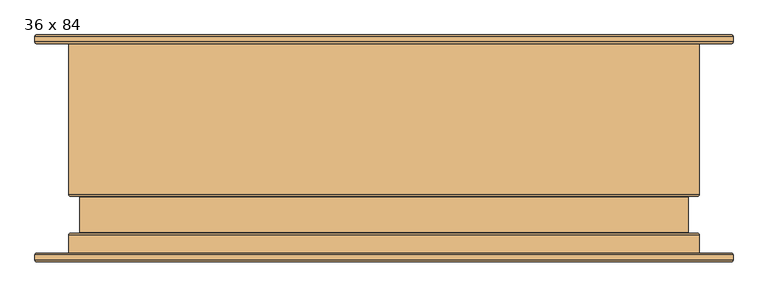
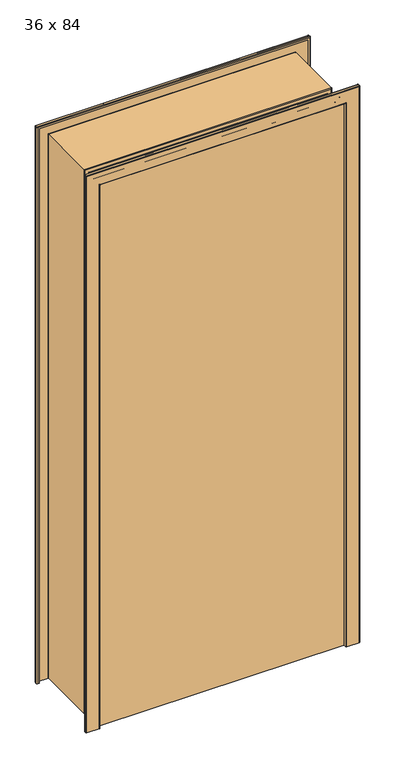
"""IFC4 building model written with IfcOpenShell, lengths in millimetres: door geometry, Door-Dunbarton_Doors-Hollow_Metal_Core : 36 x 84."""

from ifc_helpers import new_model, si_unit, frame, origin, origin_with_axes, place, context, project, spatial, polyline, circle_curve, ellipse_curve, outline, extrude, source, transform, mapped, element, save
from ifc_brep_helpers import plane_surface, cylinder_surface, revolved_surface, advanced_brep


def door_36_x_84_2b1949fa(model_context):
    return source(origin(), model_context, "Body", "SolidModel", [
        advanced_brep(
        [(-505.42825, 152.4635, 0.0), (-508.0, 155.03525, 0.0), (-508.0, 162.56, 0.0), (-505.42825, 165.13175, 0.0), (-459.77175, 165.13175, 0.0), (-457.2, 162.56, 0.0), (-457.2, -67.21475, 0.0), (-456.184, -68.23075, 0.0), (-443.89675, -68.23075, 0.0), (-441.325, -70.8025, 0.0), (-441.325, -122.5931, 0.0), (-443.89675, -125.16485, 0.0), (-456.184, -125.16485, 0.0), (-457.2, -126.18085, 0.0), (-457.2, -162.4965, 0.0), (-459.77175, -165.06825, 0.0), (-505.42825, -165.06825, 0.0), (-508.0, -162.4965, 0.0), (-508.0, -154.97175, 0.0), (-505.42825, -152.4, 0.0), (-500.0625, -152.4, 0.0), (-500.0625, -153.95575, 0.0), (-505.42825, -153.95575, 0.0), (-506.44425, -154.97175, 0.0), (-506.44425, -162.4965, 0.0), (-505.42825, -163.5125, 0.0), (-459.77175, -163.5125, 0.0), (-458.75575, -162.4965, 0.0), (-458.75575, -126.18085, 0.0), (-456.184, -123.6091, 0.0), (-443.89675, -123.6091, 0.0), (-442.88075, -122.5931, 0.0), (-442.88075, -70.8025, 0.0), (-443.89675, -69.7865, 0.0), (-456.184, -69.7865, 0.0), (-458.75575, -67.21475, 0.0), (-458.75575, 162.56, 0.0), (-459.77175, 163.576, 0.0), (-505.42825, 163.576, 0.0), (-506.44425, 162.56, 0.0), (-506.44425, 155.03525, 0.0), (-505.42825, 154.01925, 0.0), (-500.0625, 154.01925, 0.0), (-500.0625, 152.4635, 0.0), (-505.42825, 152.4635, 2181.82825), (-508.0, 155.03525, 2184.4), (-508.0, 162.56, 2184.4), (-505.42825, 165.13175, 2181.82825), (505.42825, 165.13175, 2181.82825), (505.42825, 165.13175, 0.0), (459.77175, 165.13175, 0.0), (459.77175, 165.13175, 2136.17175), (-459.77175, 165.13175, 2136.17175), (-457.2, 162.56, 2133.6), (-457.2, -67.21475, 2133.6), (-456.184, -68.23075, 2132.584), (456.184, -68.23075, 2132.584), (456.184, -68.23075, 0.0), (443.89675, -68.23075, 0.0), (443.89675, -68.23075, 2120.29675), (-443.89675, -68.23075, 2120.29675), (-441.325, -70.8025, 2117.725), (-441.325, -122.5931, 2117.725), (-443.89675, -125.16485, 2120.29675), (443.89675, -125.16485, 2120.29675), (443.89675, -125.16485, 0.0), (456.184, -125.16485, 0.0), (456.184, -125.16485, 2132.584), (-456.184, -125.16485, 2132.584), (-457.2, -126.18085, 2133.6), (-457.2, -162.4965, 2133.6), (-459.77175, -165.06825, 2136.17175), (459.77175, -165.06825, 2136.17175), (459.77175, -165.06825, 0.0), (505.42825, -165.06825, 0.0), (505.42825, -165.06825, 2181.82825), (-505.42825, -165.06825, 2181.82825), (-508.0, -162.4965, 2184.4), (-508.0, -154.97175, 2184.4), (-505.42825, -152.4, 2181.82825), (505.42825, -152.4, 2181.82825), (505.42825, -152.4, 0.0), (500.0625, -152.4, 0.0), (500.0625, -152.4, 2176.4625), (-500.0625, -152.4, 2176.4625), (-500.0625, -153.95575, 2176.4625), (500.0625, -153.95575, 2176.4625), (500.0625, -153.95575, 0.0), (505.42825, -153.95575, 0.0), (505.42825, -153.95575, 2181.82825), (-505.42825, -153.95575, 2181.82825), (-506.44425, -154.97175, 2182.84425), (-506.44425, -162.4965, 2182.84425), (-505.42825, -163.5125, 2181.82825), (505.42825, -163.5125, 2181.82825), (505.42825, -163.5125, 0.0), (459.77175, -163.5125, 0.0), (459.77175, -163.5125, 2136.17175), (-459.77175, -163.5125, 2136.17175), (-458.75575, -162.4965, 2135.15575), (-458.75575, -126.18085, 2135.15575), (-456.184, -123.6091, 2132.584), (456.184, -123.6091, 2132.584), (456.184, -123.6091, 0.0), (443.89675, -123.6091, 0.0), (443.89675, -123.6091, 2120.29675), (-443.89675, -123.6091, 2120.29675), (-442.88075, -122.5931, 2119.28075), (-442.88075, -70.8025, 2119.28075), (-443.89675, -69.7865, 2120.29675), (443.89675, -69.7865, 2120.29675), (443.89675, -69.7865, 0.0), (456.184, -69.7865, 0.0), (456.184, -69.7865, 2132.584), (-456.184, -69.7865, 2132.584), (-458.75575, -67.21475, 2135.15575), (-458.75575, 162.56, 2135.15575), (-459.77175, 163.576, 2136.17175), (459.77175, 163.576, 2136.17175), (459.77175, 163.576, 0.0), (505.42825, 163.576, 0.0), (505.42825, 163.576, 2181.82825), (-505.42825, 163.576, 2181.82825), (-506.44425, 162.56, 2182.84425), (-506.44425, 155.03525, 2182.84425), (-505.42825, 154.01925, 2181.82825), (505.42825, 154.01925, 2181.82825), (505.42825, 154.01925, 0.0), (500.0625, 154.01925, 0.0), (500.0625, 154.01925, 2176.4625), (-500.0625, 154.01925, 2176.4625), (-500.0625, 152.4635, 2176.4625), (500.0625, 152.4635, 2176.4625), (500.0625, 152.4635, 0.0), (505.42825, 152.4635, 0.0), (505.42825, 152.4635, 2181.82825), (508.0, 155.03525, 2184.4), (508.0, 162.56, 2184.4), (457.2, 162.56, 2133.6), (457.2, -67.21475, 2133.6), (441.325, -70.8025, 2117.725), (441.325, -122.5931, 2117.725), (457.2, -126.18085, 2133.6), (457.2, -162.4965, 2133.6), (508.0, -162.4965, 2184.4), (508.0, -154.97175, 2184.4), (506.44425, -154.97175, 2182.84425), (506.44425, -162.4965, 2182.84425), (458.75575, -162.4965, 2135.15575), (458.75575, -126.18085, 2135.15575), (442.88075, -122.5931, 2119.28075), (442.88075, -70.8025, 2119.28075), (458.75575, -67.21475, 2135.15575), (458.75575, 162.56, 2135.15575), (506.44425, 162.56, 2182.84425), (506.44425, 155.03525, 2182.84425), (506.44425, 155.03525, 0.0), (506.44425, 162.56, 0.0), (458.75575, 162.56, 0.0), (458.75575, -67.21475, 0.0), (442.88075, -70.8025, 0.0), (442.88075, -122.5931, 0.0), (458.75575, -126.18085, 0.0), (458.75575, -162.4965, 0.0), (506.44425, -162.4965, 0.0), (506.44425, -154.97175, 0.0), (508.0, -154.97175, 0.0), (508.0, -162.4965, 0.0), (457.2, -162.4965, 0.0), (457.2, -126.18085, 0.0), (441.325, -122.5931, 0.0), (441.325, -70.8025, 0.0), (457.2, -67.21475, 0.0), (457.2, 162.56, 0.0), (508.0, 162.56, 0.0), (508.0, 155.03525, 0.0)],
        [
            (0, 1, circle_curve(frame((-505.42825, 155.03525, 0.0), z_axis=(0.0, 0.0, -1.0), x_axis=(0.0, -1.0, 0.0)), 2.57175)),
            (1, 2),
            (2, 3, circle_curve(frame((-505.42825, 162.56, 0.0), z_axis=(0.0, 0.0, -1.0), x_axis=(0.0, -1.0, 0.0)), 2.57175)),
            (3, 4),
            (4, 5, circle_curve(frame((-459.77175, 162.56, 0.0), z_axis=(0.0, 0.0, -1.0), x_axis=(0.0, -1.0, 0.0)), 2.57175)),
            (5, 6),
            (6, 7, circle_curve(frame((-456.184, -67.21475, 0.0), z_axis=(0.0, 0.0, 1.0), x_axis=(0.0, -1.0, 0.0)), 1.016)),
            (7, 8),
            (8, 9, circle_curve(frame((-443.89675, -70.8025, 0.0), z_axis=(0.0, 0.0, -1.0), x_axis=(0.0, -1.0, 0.0)), 2.57175)),
            (9, 10),
            (10, 11, circle_curve(frame((-443.89675, -122.5931, 0.0), z_axis=(0.0, 0.0, -1.0), x_axis=(0.0, -1.0, 0.0)), 2.57175)),
            (11, 12),
            (12, 13, circle_curve(frame((-456.184, -126.18085, 0.0), z_axis=(0.0, 0.0, 1.0), x_axis=(0.0, -1.0, 0.0)), 1.016)),
            (13, 14),
            (14, 15, circle_curve(frame((-459.77175, -162.4965, 0.0), z_axis=(0.0, 0.0, -1.0), x_axis=(0.0, -1.0, 0.0)), 2.57175)),
            (15, 16),
            (16, 17, circle_curve(frame((-505.42825, -162.4965, 0.0), z_axis=(0.0, 0.0, -1.0), x_axis=(0.0, -1.0, 0.0)), 2.57175)),
            (17, 18),
            (18, 19, circle_curve(frame((-505.42825, -154.97175, 0.0), z_axis=(0.0, 0.0, -1.0), x_axis=(0.0, -1.0, 0.0)), 2.57175)),
            (19, 20),
            (20, 21),
            (21, 22),
            (22, 23, circle_curve(frame((-505.42825, -154.97175, 0.0), z_axis=(0.0, 0.0, 1.0), x_axis=(0.0, -1.0, 0.0)), 1.016)),
            (23, 24),
            (24, 25, circle_curve(frame((-505.42825, -162.4965, 0.0), z_axis=(0.0, 0.0, 1.0), x_axis=(0.0, -1.0, 0.0)), 1.016)),
            (25, 26),
            (26, 27, circle_curve(frame((-459.77175, -162.4965, 0.0), z_axis=(0.0, 0.0, 1.0), x_axis=(0.0, -1.0, 0.0)), 1.016)),
            (27, 28),
            (28, 29, circle_curve(frame((-456.184, -126.18085, 0.0), z_axis=(0.0, 0.0, -1.0), x_axis=(0.0, -1.0, 0.0)), 2.57175)),
            (29, 30),
            (30, 31, circle_curve(frame((-443.89675, -122.5931, 0.0), z_axis=(0.0, 0.0, 1.0), x_axis=(0.0, -1.0, 0.0)), 1.016)),
            (31, 32),
            (32, 33, circle_curve(frame((-443.89675, -70.8025, 0.0), z_axis=(0.0, 0.0, 1.0), x_axis=(0.0, -1.0, 0.0)), 1.016)),
            (33, 34),
            (34, 35, circle_curve(frame((-456.184, -67.21475, 0.0), z_axis=(0.0, 0.0, -1.0), x_axis=(0.0, -1.0, 0.0)), 2.57175)),
            (35, 36),
            (36, 37, circle_curve(frame((-459.77175, 162.56, 0.0), z_axis=(0.0, 0.0, 1.0), x_axis=(0.0, -1.0, 0.0)), 1.016)),
            (37, 38),
            (38, 39, circle_curve(frame((-505.42825, 162.56, 0.0), z_axis=(0.0, 0.0, 1.0), x_axis=(0.0, -1.0, 0.0)), 1.016)),
            (39, 40),
            (40, 41, circle_curve(frame((-505.42825, 155.03525, 0.0), z_axis=(0.0, 0.0, 1.0), x_axis=(0.0, -1.0, 0.0)), 1.016)),
            (41, 42),
            (42, 43),
            (43, 0),
            (0, 44),
            (44, 45, ellipse_curve(frame((-505.42825, 155.03525, 2181.82825), z_axis=(-0.7071067811865475, 0.0, -0.7071067811865475), x_axis=(0.7071067811865474, 0.0, -0.7071067811865476)), 3.6370037, 2.57175)),
            (45, 1),
            (45, 46),
            (46, 2),
            (46, 47, ellipse_curve(frame((-505.42825, 162.56, 2181.82825), z_axis=(-0.7071067811865475, 0.0, -0.7071067811865475), x_axis=(0.7071067811865474, 0.0, -0.7071067811865476)), 3.6370037, 2.57175)),
            (47, 3),
            (47, 48),
            (48, 49),
            (49, 50),
            (50, 51),
            (51, 52),
            (52, 4),
            (52, 53, ellipse_curve(frame((-459.77175, 162.56, 2136.17175), z_axis=(-0.7071067811865475, 0.0, -0.7071067811865475), x_axis=(0.7071067811865474, 0.0, -0.7071067811865476)), 3.6370037, 2.57175)),
            (53, 5),
            (53, 54),
            (54, 6),
            (54, 55, ellipse_curve(frame((-456.184, -67.21475, 2132.584), z_axis=(0.7071067811865475, 0.0, 0.7071067811865475), x_axis=(-0.7071067811865474, 0.0, 0.7071067811865476)), 1.436841, 1.016)),
            (55, 7),
            (55, 56),
            (56, 57),
            (57, 58),
            (58, 59),
            (59, 60),
            (60, 8),
            (60, 61, ellipse_curve(frame((-443.89675, -70.8025, 2120.29675), z_axis=(-0.7071067811865475, 0.0, -0.7071067811865475), x_axis=(0.7071067811865474, 0.0, -0.7071067811865476)), 3.6370037, 2.57175)),
            (61, 9),
            (61, 62),
            (62, 10),
            (62, 63, ellipse_curve(frame((-443.89675, -122.5931, 2120.29675), z_axis=(-0.7071067811865475, 0.0, -0.7071067811865475), x_axis=(0.7071067811865474, 0.0, -0.7071067811865476)), 3.6370037, 2.57175)),
            (63, 11),
            (63, 64),
            (64, 65),
            (65, 66),
            (66, 67),
            (67, 68),
            (68, 12),
            (68, 69, ellipse_curve(frame((-456.184, -126.18085, 2132.584), z_axis=(0.7071067811865475, 0.0, 0.7071067811865475), x_axis=(-0.7071067811865474, 0.0, 0.7071067811865476)), 1.436841, 1.016)),
            (69, 13),
            (69, 70),
            (70, 14),
            (70, 71, ellipse_curve(frame((-459.77175, -162.4965, 2136.17175), z_axis=(-0.7071067811865475, 0.0, -0.7071067811865475), x_axis=(0.7071067811865474, 0.0, -0.7071067811865476)), 3.6370037, 2.57175)),
            (71, 15),
            (71, 72),
            (72, 73),
            (73, 74),
            (74, 75),
            (75, 76),
            (76, 16),
            (76, 77, ellipse_curve(frame((-505.42825, -162.4965, 2181.82825), z_axis=(-0.7071067811865475, 0.0, -0.7071067811865475), x_axis=(0.7071067811865474, 0.0, -0.7071067811865476)), 3.6370037, 2.57175)),
            (77, 17),
            (77, 78),
            (78, 18),
            (78, 79, ellipse_curve(frame((-505.42825, -154.97175, 2181.82825), z_axis=(-0.7071067811865475, 0.0, -0.7071067811865475), x_axis=(0.7071067811865474, 0.0, -0.7071067811865476)), 3.6370037, 2.57175)),
            (79, 19),
            (79, 80),
            (80, 81),
            (81, 82),
            (82, 83),
            (83, 84),
            (84, 20),
            (84, 85),
            (85, 21),
            (85, 86),
            (86, 87),
            (87, 88),
            (88, 89),
            (89, 90),
            (90, 22),
            (90, 91, ellipse_curve(frame((-505.42825, -154.97175, 2181.82825), z_axis=(0.7071067811865475, 0.0, 0.7071067811865475), x_axis=(-0.7071067811865474, 0.0, 0.7071067811865476)), 1.436841, 1.016)),
            (91, 23),
            (91, 92),
            (92, 24),
            (92, 93, ellipse_curve(frame((-505.42825, -162.4965, 2181.82825), z_axis=(0.7071067811865475, 0.0, 0.7071067811865475), x_axis=(-0.7071067811865474, 0.0, 0.7071067811865476)), 1.436841, 1.016)),
            (93, 25),
            (93, 94),
            (94, 95),
            (95, 96),
            (96, 97),
            (97, 98),
            (98, 26),
            (98, 99, ellipse_curve(frame((-459.77175, -162.4965, 2136.17175), z_axis=(0.7071067811865475, 0.0, 0.7071067811865475), x_axis=(-0.7071067811865474, 0.0, 0.7071067811865476)), 1.436841, 1.016)),
            (99, 27),
            (99, 100),
            (100, 28),
            (100, 101, ellipse_curve(frame((-456.184, -126.18085, 2132.584), z_axis=(-0.7071067811865475, 0.0, -0.7071067811865475), x_axis=(0.7071067811865474, 0.0, -0.7071067811865476)), 3.6370037, 2.57175)),
            (101, 29),
            (101, 102),
            (102, 103),
            (103, 104),
            (104, 105),
            (105, 106),
            (106, 30),
            (106, 107, ellipse_curve(frame((-443.89675, -122.5931, 2120.29675), z_axis=(0.7071067811865475, 0.0, 0.7071067811865475), x_axis=(-0.7071067811865474, 0.0, 0.7071067811865476)), 1.436841, 1.016)),
            (107, 31),
            (107, 108),
            (108, 32),
            (108, 109, ellipse_curve(frame((-443.89675, -70.8025, 2120.29675), z_axis=(0.7071067811865475, 0.0, 0.7071067811865475), x_axis=(-0.7071067811865474, 0.0, 0.7071067811865476)), 1.436841, 1.016)),
            (109, 33),
            (109, 110),
            (110, 111),
            (111, 112),
            (112, 113),
            (113, 114),
            (114, 34),
            (114, 115, ellipse_curve(frame((-456.184, -67.21475, 2132.584), z_axis=(-0.7071067811865475, 0.0, -0.7071067811865475), x_axis=(0.7071067811865474, 0.0, -0.7071067811865476)), 3.6370037, 2.57175)),
            (115, 35),
            (115, 116),
            (116, 36),
            (116, 117, ellipse_curve(frame((-459.77175, 162.56, 2136.17175), z_axis=(0.7071067811865475, 0.0, 0.7071067811865475), x_axis=(-0.7071067811865474, 0.0, 0.7071067811865476)), 1.436841, 1.016)),
            (117, 37),
            (117, 118),
            (118, 119),
            (119, 120),
            (120, 121),
            (121, 122),
            (122, 38),
            (122, 123, ellipse_curve(frame((-505.42825, 162.56, 2181.82825), z_axis=(0.7071067811865475, 0.0, 0.7071067811865475), x_axis=(-0.7071067811865474, 0.0, 0.7071067811865476)), 1.436841, 1.016)),
            (123, 39),
            (123, 124),
            (124, 40),
            (124, 125, ellipse_curve(frame((-505.42825, 155.03525, 2181.82825), z_axis=(0.7071067811865475, 0.0, 0.7071067811865475), x_axis=(-0.7071067811865474, 0.0, 0.7071067811865476)), 1.436841, 1.016)),
            (125, 41),
            (125, 126),
            (126, 127),
            (127, 128),
            (128, 129),
            (129, 130),
            (130, 42),
            (130, 131),
            (131, 43),
            (131, 132),
            (132, 133),
            (133, 134),
            (134, 135),
            (135, 44),
            (135, 136, ellipse_curve(frame((505.42825, 155.03525, 2181.82825), z_axis=(-0.7071067811865475, 0.0, 0.7071067811865475), x_axis=(-0.7071067811865476, 0.0, -0.7071067811865474)), 3.6370037, 2.57175)),
            (136, 45),
            (136, 137),
            (137, 46),
            (137, 48, ellipse_curve(frame((505.42825, 162.56, 2181.82825), z_axis=(-0.7071067811865475, 0.0, 0.7071067811865475), x_axis=(-0.7071067811865476, 0.0, -0.7071067811865474)), 3.6370037, 2.57175)),
            (51, 138, ellipse_curve(frame((459.77175, 162.56, 2136.17175), z_axis=(-0.7071067811865475, 0.0, 0.7071067811865475), x_axis=(-0.7071067811865476, 0.0, -0.7071067811865474)), 3.6370037, 2.57175)),
            (138, 53),
            (138, 139),
            (139, 54),
            (139, 56, ellipse_curve(frame((456.184, -67.21475, 2132.584), z_axis=(0.7071067811865475, 0.0, -0.7071067811865475), x_axis=(0.7071067811865476, 0.0, 0.7071067811865474)), 1.436841, 1.016)),
            (59, 140, ellipse_curve(frame((443.89675, -70.8025, 2120.29675), z_axis=(-0.7071067811865475, 0.0, 0.7071067811865475), x_axis=(-0.7071067811865476, 0.0, -0.7071067811865474)), 3.6370037, 2.57175)),
            (140, 61),
            (140, 141),
            (141, 62),
            (141, 64, ellipse_curve(frame((443.89675, -122.5931, 2120.29675), z_axis=(-0.7071067811865475, 0.0, 0.7071067811865475), x_axis=(-0.7071067811865476, 0.0, -0.7071067811865474)), 3.6370037, 2.57175)),
            (67, 142, ellipse_curve(frame((456.184, -126.18085, 2132.584), z_axis=(0.7071067811865475, 0.0, -0.7071067811865475), x_axis=(0.7071067811865476, 0.0, 0.7071067811865474)), 1.436841, 1.016)),
            (142, 69),
            (142, 143),
            (143, 70),
            (143, 72, ellipse_curve(frame((459.77175, -162.4965, 2136.17175), z_axis=(-0.7071067811865475, 0.0, 0.7071067811865475), x_axis=(-0.7071067811865476, 0.0, -0.7071067811865474)), 3.6370037, 2.57175)),
            (75, 144, ellipse_curve(frame((505.42825, -162.4965, 2181.82825), z_axis=(-0.7071067811865475, 0.0, 0.7071067811865475), x_axis=(-0.7071067811865476, 0.0, -0.7071067811865474)), 3.6370037, 2.57175)),
            (144, 77),
            (144, 145),
            (145, 78),
            (145, 80, ellipse_curve(frame((505.42825, -154.97175, 2181.82825), z_axis=(-0.7071067811865475, 0.0, 0.7071067811865475), x_axis=(-0.7071067811865476, 0.0, -0.7071067811865474)), 3.6370037, 2.57175)),
            (83, 86),
            (89, 146, ellipse_curve(frame((505.42825, -154.97175, 2181.82825), z_axis=(0.7071067811865475, 0.0, -0.7071067811865475), x_axis=(0.7071067811865476, 0.0, 0.7071067811865474)), 1.436841, 1.016)),
            (146, 91),
            (146, 147),
            (147, 92),
            (147, 94, ellipse_curve(frame((505.42825, -162.4965, 2181.82825), z_axis=(0.7071067811865475, 0.0, -0.7071067811865475), x_axis=(0.7071067811865476, 0.0, 0.7071067811865474)), 1.436841, 1.016)),
            (97, 148, ellipse_curve(frame((459.77175, -162.4965, 2136.17175), z_axis=(0.7071067811865475, 0.0, -0.7071067811865475), x_axis=(0.7071067811865476, 0.0, 0.7071067811865474)), 1.436841, 1.016)),
            (148, 99),
            (148, 149),
            (149, 100),
            (149, 102, ellipse_curve(frame((456.184, -126.18085, 2132.584), z_axis=(-0.7071067811865475, 0.0, 0.7071067811865475), x_axis=(-0.7071067811865476, 0.0, -0.7071067811865474)), 3.6370037, 2.57175)),
            (105, 150, ellipse_curve(frame((443.89675, -122.5931, 2120.29675), z_axis=(0.7071067811865475, 0.0, -0.7071067811865475), x_axis=(0.7071067811865476, 0.0, 0.7071067811865474)), 1.436841, 1.016)),
            (150, 107),
            (150, 151),
            (151, 108),
            (151, 110, ellipse_curve(frame((443.89675, -70.8025, 2120.29675), z_axis=(0.7071067811865475, 0.0, -0.7071067811865475), x_axis=(0.7071067811865476, 0.0, 0.7071067811865474)), 1.436841, 1.016)),
            (113, 152, ellipse_curve(frame((456.184, -67.21475, 2132.584), z_axis=(-0.7071067811865475, 0.0, 0.7071067811865475), x_axis=(-0.7071067811865476, 0.0, -0.7071067811865474)), 3.6370037, 2.57175)),
            (152, 115),
            (152, 153),
            (153, 116),
            (153, 118, ellipse_curve(frame((459.77175, 162.56, 2136.17175), z_axis=(0.7071067811865475, 0.0, -0.7071067811865475), x_axis=(0.7071067811865476, 0.0, 0.7071067811865474)), 1.436841, 1.016)),
            (121, 154, ellipse_curve(frame((505.42825, 162.56, 2181.82825), z_axis=(0.7071067811865475, 0.0, -0.7071067811865475), x_axis=(0.7071067811865476, 0.0, 0.7071067811865474)), 1.436841, 1.016)),
            (154, 123),
            (154, 155),
            (155, 124),
            (155, 126, ellipse_curve(frame((505.42825, 155.03525, 2181.82825), z_axis=(0.7071067811865475, 0.0, -0.7071067811865475), x_axis=(0.7071067811865476, 0.0, 0.7071067811865474)), 1.436841, 1.016)),
            (129, 132),
            (133, 128),
            (127, 156, circle_curve(frame((505.42825, 155.03525, 0.0), z_axis=(0.0, 0.0, 1.0), x_axis=(0.0, -1.0, 0.0)), 1.016)),
            (156, 157),
            (157, 120, circle_curve(frame((505.42825, 162.56, 0.0), z_axis=(0.0, 0.0, 1.0), x_axis=(0.0, -1.0, 0.0)), 1.016)),
            (119, 158, circle_curve(frame((459.77175, 162.56, 0.0), z_axis=(0.0, 0.0, 1.0), x_axis=(0.0, -1.0, 0.0)), 1.016)),
            (158, 159),
            (159, 112, circle_curve(frame((456.184, -67.21475, 0.0), z_axis=(0.0, 0.0, -1.0), x_axis=(0.0, -1.0, 0.0)), 2.57175)),
            (111, 160, circle_curve(frame((443.89675, -70.8025, 0.0), z_axis=(0.0, 0.0, 1.0), x_axis=(0.0, -1.0, 0.0)), 1.016)),
            (160, 161),
            (161, 104, circle_curve(frame((443.89675, -122.5931, 0.0), z_axis=(0.0, 0.0, 1.0), x_axis=(0.0, -1.0, 0.0)), 1.016)),
            (103, 162, circle_curve(frame((456.184, -126.18085, 0.0), z_axis=(0.0, 0.0, -1.0), x_axis=(0.0, -1.0, 0.0)), 2.57175)),
            (162, 163),
            (163, 96, circle_curve(frame((459.77175, -162.4965, 0.0), z_axis=(0.0, 0.0, 1.0), x_axis=(0.0, -1.0, 0.0)), 1.016)),
            (95, 164, circle_curve(frame((505.42825, -162.4965, 0.0), z_axis=(0.0, 0.0, 1.0), x_axis=(0.0, -1.0, 0.0)), 1.016)),
            (164, 165),
            (165, 88, circle_curve(frame((505.42825, -154.97175, 0.0), z_axis=(0.0, 0.0, 1.0), x_axis=(0.0, -1.0, 0.0)), 1.016)),
            (87, 82),
            (81, 166, circle_curve(frame((505.42825, -154.97175, 0.0), z_axis=(0.0, 0.0, -1.0), x_axis=(0.0, -1.0, 0.0)), 2.57175)),
            (166, 167),
            (167, 74, circle_curve(frame((505.42825, -162.4965, 0.0), z_axis=(0.0, 0.0, -1.0), x_axis=(0.0, -1.0, 0.0)), 2.57175)),
            (73, 168, circle_curve(frame((459.77175, -162.4965, 0.0), z_axis=(0.0, 0.0, -1.0), x_axis=(0.0, -1.0, 0.0)), 2.57175)),
            (168, 169),
            (169, 66, circle_curve(frame((456.184, -126.18085, 0.0), z_axis=(0.0, 0.0, 1.0), x_axis=(0.0, -1.0, 0.0)), 1.016)),
            (65, 170, circle_curve(frame((443.89675, -122.5931, 0.0), z_axis=(0.0, 0.0, -1.0), x_axis=(0.0, -1.0, 0.0)), 2.57175)),
            (170, 171),
            (171, 58, circle_curve(frame((443.89675, -70.8025, 0.0), z_axis=(0.0, 0.0, -1.0), x_axis=(0.0, -1.0, 0.0)), 2.57175)),
            (57, 172, circle_curve(frame((456.184, -67.21475, 0.0), z_axis=(0.0, 0.0, 1.0), x_axis=(0.0, -1.0, 0.0)), 1.016)),
            (172, 173),
            (173, 50, circle_curve(frame((459.77175, 162.56, 0.0), z_axis=(0.0, 0.0, -1.0), x_axis=(0.0, -1.0, 0.0)), 2.57175)),
            (49, 174, circle_curve(frame((505.42825, 162.56, 0.0), z_axis=(0.0, 0.0, -1.0), x_axis=(0.0, -1.0, 0.0)), 2.57175)),
            (174, 175),
            (175, 134, circle_curve(frame((505.42825, 155.03525, 0.0), z_axis=(0.0, 0.0, -1.0), x_axis=(0.0, -1.0, 0.0)), 2.57175)),
            (175, 136),
            (174, 137),
            (173, 138),
            (172, 139),
            (171, 140),
            (170, 141),
            (169, 142),
            (168, 143),
            (167, 144),
            (166, 145),
            (165, 146),
            (164, 147),
            (163, 148),
            (162, 149),
            (161, 150),
            (160, 151),
            (159, 152),
            (158, 153),
            (157, 154),
            (156, 155),
        ],
        [
            plane_surface(frame((-468.3125, -152.4, 0.0), z_axis=(0.0, 0.0, -1.0), x_axis=(1.0, 0.0, 0.0))),
            cylinder_surface(frame((-505.42825, 155.03525, 0.0), z_axis=(0.0, 0.0, -1.0), x_axis=(0.0, -1.0, 0.0)), 2.57175),
            plane_surface(frame((-508.0, 155.03525, 0.0), z_axis=(-1.0, 0.0, 0.0), x_axis=(0.0, 0.0, 1.0))),
            cylinder_surface(frame((-505.42825, 162.56, 0.0), z_axis=(0.0, 0.0, -1.0), x_axis=(0.0, -1.0, 0.0)), 2.57175),
            plane_surface(frame((-505.42825, 165.13175, 0.0), z_axis=(0.0, 1.0, 0.0), x_axis=(0.0, 0.0, 1.0))),
            cylinder_surface(frame((-459.77175, 162.56, 0.0), z_axis=(0.0, 0.0, -1.0), x_axis=(0.0, -1.0, 0.0)), 2.57175),
            plane_surface(frame((-457.2, 162.56, 0.0), z_axis=(1.0, 0.0, 0.0), x_axis=(0.0, 0.0, 1.0))),
            revolved_surface(polyline([(-456.184, -68.23075, 2133.600000014587), (-456.184, -68.23075, 0.0)]), (-456.184, -67.21475, 0.0), (0.0, 0.0, 1.0)),
            plane_surface(frame((-456.184, -68.23075, 0.0), z_axis=(0.0, 1.0, 0.0), x_axis=(0.0, 0.0, 1.0))),
            cylinder_surface(frame((-443.89675, -70.8025, 0.0), z_axis=(0.0, 0.0, -1.0), x_axis=(0.0, -1.0, 0.0)), 2.57175),
            plane_surface(frame((-441.325, -70.8025, 0.0), z_axis=(1.0, 0.0, 0.0), x_axis=(0.0, 0.0, 1.0))),
            cylinder_surface(frame((-443.89675, -122.5931, 0.0), z_axis=(0.0, 0.0, -1.0), x_axis=(0.0, -1.0, 0.0)), 2.57175),
            plane_surface(frame((-443.89675, -125.16485, 0.0), z_axis=(0.0, -1.0, 0.0), x_axis=(0.0, 0.0, 1.0))),
            revolved_surface(polyline([(-456.184, -127.19685000000001, 2133.600000014587), (-456.184, -127.19685000000001, 0.0)]), (-456.184, -126.18085, 0.0), (0.0, 0.0, 1.0)),
            plane_surface(frame((-457.2, -126.18085, 0.0), z_axis=(1.0, 0.0, 0.0), x_axis=(0.0, 0.0, 1.0))),
            cylinder_surface(frame((-459.77175, -162.4965, 0.0), z_axis=(0.0, 0.0, -1.0), x_axis=(0.0, -1.0, 0.0)), 2.57175),
            plane_surface(frame((-459.77175, -165.06825, 0.0), z_axis=(0.0, -1.0, 0.0), x_axis=(0.0, 0.0, 1.0))),
            cylinder_surface(frame((-505.42825, -162.4965, 0.0), z_axis=(0.0, 0.0, -1.0), x_axis=(0.0, -1.0, 0.0)), 2.57175),
            plane_surface(frame((-508.0, -162.4965, 0.0), z_axis=(-1.0, 0.0, 0.0), x_axis=(0.0, 0.0, 1.0))),
            cylinder_surface(frame((-505.42825, -154.97175, 0.0), z_axis=(0.0, 0.0, -1.0), x_axis=(0.0, -1.0, 0.0)), 2.57175),
            plane_surface(frame((-505.42825, -152.4, 0.0), z_axis=(0.0, 1.0, 0.0), x_axis=(0.0, 0.0, 1.0))),
            plane_surface(frame((-500.0625, -152.4, 0.0), z_axis=(1.0, 0.0, 0.0), x_axis=(0.0, 0.0, 1.0))),
            plane_surface(frame((-500.0625, -153.95575, 0.0), z_axis=(0.0, -1.0, 0.0), x_axis=(0.0, 0.0, 1.0))),
            revolved_surface(polyline([(-505.42825, -155.98774999999998, 2182.844250014587), (-505.42825, -155.98774999999998, 0.0)]), (-505.42825, -154.97175, 0.0), (0.0, 0.0, 1.0)),
            plane_surface(frame((-506.44425, -154.97175, 0.0), z_axis=(1.0, 0.0, 0.0), x_axis=(0.0, 0.0, 1.0))),
            revolved_surface(polyline([(-505.42825, -163.5125, 2182.844250014587), (-505.42825, -163.5125, 0.0)]), (-505.42825, -162.4965, 0.0), (0.0, 0.0, 1.0)),
            plane_surface(frame((-505.42825, -163.5125, 0.0), z_axis=(0.0, 1.0, 0.0), x_axis=(0.0, 0.0, 1.0))),
            revolved_surface(polyline([(-459.77175, -163.5125, 2137.187750014587), (-459.77175, -163.5125, 0.0)]), (-459.77175, -162.4965, 0.0), (0.0, 0.0, 1.0)),
            plane_surface(frame((-458.75575, -162.4965, 0.0), z_axis=(-1.0, 0.0, 0.0), x_axis=(0.0, 0.0, 1.0))),
            cylinder_surface(frame((-456.184, -126.18085, 0.0), z_axis=(0.0, 0.0, -1.0), x_axis=(0.0, -1.0, 0.0)), 2.57175),
            plane_surface(frame((-456.184, -123.6091, 0.0), z_axis=(0.0, 1.0, 0.0), x_axis=(0.0, 0.0, 1.0))),
            revolved_surface(polyline([(-443.89675, -123.60910000000001, 2121.312750014587), (-443.89675, -123.60910000000001, 0.0)]), (-443.89675, -122.5931, 0.0), (0.0, 0.0, 1.0)),
            plane_surface(frame((-442.88075, -122.5931, 0.0), z_axis=(-1.0, 0.0, 0.0), x_axis=(0.0, 0.0, 1.0))),
            revolved_surface(polyline([(-443.89675, -71.8185, 2121.312750014587), (-443.89675, -71.8185, 0.0)]), (-443.89675, -70.8025, 0.0), (0.0, 0.0, 1.0)),
            plane_surface(frame((-443.89675, -69.7865, 0.0), z_axis=(0.0, -1.0, 0.0), x_axis=(0.0, 0.0, 1.0))),
            cylinder_surface(frame((-456.184, -67.21475, 0.0), z_axis=(0.0, 0.0, -1.0), x_axis=(0.0, -1.0, 0.0)), 2.57175),
            plane_surface(frame((-458.75575, -67.21475, 0.0), z_axis=(-1.0, 0.0, 0.0), x_axis=(0.0, 0.0, 1.0))),
            revolved_surface(polyline([(-459.77175, 161.544, 2137.187750014587), (-459.77175, 161.544, 0.0)]), (-459.77175, 162.56, 0.0), (0.0, 0.0, 1.0)),
            plane_surface(frame((-459.77175, 163.576, 0.0), z_axis=(0.0, -1.0, 0.0), x_axis=(0.0, 0.0, 1.0))),
            revolved_surface(polyline([(-505.42825, 161.544, 2182.844250014587), (-505.42825, 161.544, 0.0)]), (-505.42825, 162.56, 0.0), (0.0, 0.0, 1.0)),
            plane_surface(frame((-506.44425, 162.56, 0.0), z_axis=(1.0, 0.0, 0.0), x_axis=(0.0, 0.0, 1.0))),
            revolved_surface(polyline([(-505.42825, 154.01925, 2182.844250014587), (-505.42825, 154.01925, 0.0)]), (-505.42825, 155.03525, 0.0), (0.0, 0.0, 1.0)),
            plane_surface(frame((-505.42825, 154.01925, 0.0), z_axis=(0.0, 1.0, 0.0), x_axis=(0.0, 0.0, 1.0))),
            plane_surface(frame((-500.0625, 154.01925, 0.0), z_axis=(1.0, 0.0, 0.0), x_axis=(0.0, 0.0, 1.0))),
            plane_surface(frame((-500.0625, 152.4635, 0.0), z_axis=(0.0, -1.0, 0.0), x_axis=(0.0, 0.0, 1.0))),
            cylinder_surface(frame((-468.3125, 155.03525, 2181.82825), z_axis=(-1.0, 0.0, 0.0), x_axis=(0.0, -1.0, 0.0)), 2.57175),
            plane_surface(frame((-508.0, 155.03525, 2184.4), z_axis=(0.0, 0.0, 1.0), x_axis=(1.0, 0.0, 0.0))),
            cylinder_surface(frame((-468.3125, 162.56, 2181.82825), z_axis=(-1.0, 0.0, 0.0), x_axis=(0.0, -1.0, 0.0)), 2.57175),
            cylinder_surface(frame((-468.3125, 162.56, 2136.17175), z_axis=(-1.0, 0.0, 0.0), x_axis=(0.0, -1.0, 0.0)), 2.57175),
            plane_surface(frame((-457.2, 162.56, 2133.6), z_axis=(0.0, 0.0, -1.0), x_axis=(1.0, 0.0, 0.0))),
            revolved_surface(polyline([(457.20000001458686, -68.23075, 2132.584), (-457.20000001458686, -68.23075, 2132.584)]), (-468.3125, -67.21475, 2132.584), (1.0, 0.0, 0.0)),
            cylinder_surface(frame((-468.3125, -70.8025, 2120.29675), z_axis=(-1.0, 0.0, 0.0), x_axis=(0.0, -1.0, 0.0)), 2.57175),
            plane_surface(frame((-441.325, -70.8025, 2117.725), z_axis=(0.0, 0.0, -1.0), x_axis=(1.0, 0.0, 0.0))),
            cylinder_surface(frame((-468.3125, -122.5931, 2120.29675), z_axis=(-1.0, 0.0, 0.0), x_axis=(0.0, -1.0, 0.0)), 2.57175),
            revolved_surface(polyline([(457.20000001458686, -127.19685000000001, 2132.584), (-457.20000001458686, -127.19685000000001, 2132.584)]), (-468.3125, -126.18085, 2132.584), (1.0, 0.0, 0.0)),
            plane_surface(frame((-457.2, -126.18085, 2133.6), z_axis=(0.0, 0.0, -1.0), x_axis=(1.0, 0.0, 0.0))),
            cylinder_surface(frame((-468.3125, -162.4965, 2136.17175), z_axis=(-1.0, 0.0, 0.0), x_axis=(0.0, -1.0, 0.0)), 2.57175),
            cylinder_surface(frame((-468.3125, -162.4965, 2181.82825), z_axis=(-1.0, 0.0, 0.0), x_axis=(0.0, -1.0, 0.0)), 2.57175),
            plane_surface(frame((-508.0, -162.4965, 2184.4), z_axis=(0.0, 0.0, 1.0), x_axis=(1.0, 0.0, 0.0))),
            cylinder_surface(frame((-468.3125, -154.97175, 2181.82825), z_axis=(-1.0, 0.0, 0.0), x_axis=(0.0, -1.0, 0.0)), 2.57175),
            plane_surface(frame((-500.0625, -152.4, 2176.4625), z_axis=(0.0, 0.0, -1.0), x_axis=(1.0, 0.0, 0.0))),
            revolved_surface(polyline([(506.4442500145868, -155.98774999999998, 2181.82825), (-506.4442500145868, -155.98774999999998, 2181.82825)]), (-468.3125, -154.97175, 2181.82825), (1.0, 0.0, 0.0)),
            plane_surface(frame((-506.44425, -154.97175, 2182.84425), z_axis=(0.0, 0.0, -1.0), x_axis=(1.0, 0.0, 0.0))),
            revolved_surface(polyline([(506.4442500145868, -163.5125, 2181.82825), (-506.4442500145868, -163.5125, 2181.82825)]), (-468.3125, -162.4965, 2181.82825), (1.0, 0.0, 0.0)),
            revolved_surface(polyline([(460.7877500145869, -163.5125, 2136.17175), (-460.78775001458683, -163.5125, 2136.17175)]), (-468.3125, -162.4965, 2136.17175), (1.0, 0.0, 0.0)),
            plane_surface(frame((-458.75575, -162.4965, 2135.15575), z_axis=(0.0, 0.0, 1.0), x_axis=(1.0, 0.0, 0.0))),
            cylinder_surface(frame((-468.3125, -126.18085, 2132.584), z_axis=(-1.0, 0.0, 0.0), x_axis=(0.0, -1.0, 0.0)), 2.57175),
            revolved_surface(polyline([(444.9127500145869, -123.60910000000001, 2120.29675), (-444.91275001458683, -123.60910000000001, 2120.29675)]), (-468.3125, -122.5931, 2120.29675), (1.0, 0.0, 0.0)),
            plane_surface(frame((-442.88075, -122.5931, 2119.28075), z_axis=(0.0, 0.0, 1.0), x_axis=(1.0, 0.0, 0.0))),
            revolved_surface(polyline([(444.9127500145869, -71.8185, 2120.29675), (-444.91275001458683, -71.8185, 2120.29675)]), (-468.3125, -70.8025, 2120.29675), (1.0, 0.0, 0.0)),
            cylinder_surface(frame((-468.3125, -67.21475, 2132.584), z_axis=(-1.0, 0.0, 0.0), x_axis=(0.0, -1.0, 0.0)), 2.57175),
            plane_surface(frame((-458.75575, -67.21475, 2135.15575), z_axis=(0.0, 0.0, 1.0), x_axis=(1.0, 0.0, 0.0))),
            revolved_surface(polyline([(460.7877500145869, 161.544, 2136.17175), (-460.78775001458683, 161.544, 2136.17175)]), (-468.3125, 162.56, 2136.17175), (1.0, 0.0, 0.0)),
            revolved_surface(polyline([(506.4442500145868, 161.544, 2181.82825), (-506.4442500145868, 161.544, 2181.82825)]), (-468.3125, 162.56, 2181.82825), (1.0, 0.0, 0.0)),
            plane_surface(frame((-506.44425, 162.56, 2182.84425), z_axis=(0.0, 0.0, -1.0), x_axis=(1.0, 0.0, 0.0))),
            revolved_surface(polyline([(506.4442500145868, 154.01925, 2181.82825), (-506.4442500145868, 154.01925, 2181.82825)]), (-468.3125, 155.03525, 2181.82825), (1.0, 0.0, 0.0)),
            plane_surface(frame((-500.0625, 154.01925, 2176.4625), z_axis=(0.0, 0.0, -1.0), x_axis=(1.0, 0.0, 0.0))),
            plane_surface(frame((468.3125, -152.4, 0.0), z_axis=(0.0, 0.0, -1.0), x_axis=(-1.0, 0.0, 0.0))),
            cylinder_surface(frame((505.42825, 155.03525, 2144.7125), z_axis=(0.0, 0.0, 1.0), x_axis=(0.0, -1.0, 0.0)), 2.57175),
            plane_surface(frame((508.0, 155.03525, 2184.4), z_axis=(1.0, 0.0, 0.0), x_axis=(0.0, 0.0, -1.0))),
            cylinder_surface(frame((505.42825, 162.56, 2144.7125), z_axis=(0.0, 0.0, 1.0), x_axis=(0.0, -1.0, 0.0)), 2.57175),
            cylinder_surface(frame((459.77175, 162.56, 2144.7125), z_axis=(0.0, 0.0, 1.0), x_axis=(0.0, -1.0, 0.0)), 2.57175),
            plane_surface(frame((457.2, 162.56, 2133.6), z_axis=(-1.0, 0.0, 0.0), x_axis=(0.0, 0.0, -1.0))),
            revolved_surface(polyline([(456.184, -68.23075, 0.0), (456.184, -68.23075, 2133.600000014587)]), (456.184, -67.21475, 2144.7125), (0.0, 0.0, -1.0)),
            cylinder_surface(frame((443.89675, -70.8025, 2144.7125), z_axis=(0.0, 0.0, 1.0), x_axis=(0.0, -1.0, 0.0)), 2.57175),
            plane_surface(frame((441.325, -70.8025, 2117.725), z_axis=(-1.0, 0.0, 0.0), x_axis=(0.0, 0.0, -1.0))),
            cylinder_surface(frame((443.89675, -122.5931, 2144.7125), z_axis=(0.0, 0.0, 1.0), x_axis=(0.0, -1.0, 0.0)), 2.57175),
            revolved_surface(polyline([(456.184, -127.19685000000001, 0.0), (456.184, -127.19685000000001, 2133.600000014587)]), (456.184, -126.18085, 2144.7125), (0.0, 0.0, -1.0)),
            plane_surface(frame((457.2, -126.18085, 2133.6), z_axis=(-1.0, 0.0, 0.0), x_axis=(0.0, 0.0, -1.0))),
            cylinder_surface(frame((459.77175, -162.4965, 2144.7125), z_axis=(0.0, 0.0, 1.0), x_axis=(0.0, -1.0, 0.0)), 2.57175),
            cylinder_surface(frame((505.42825, -162.4965, 2144.7125), z_axis=(0.0, 0.0, 1.0), x_axis=(0.0, -1.0, 0.0)), 2.57175),
            plane_surface(frame((508.0, -162.4965, 2184.4), z_axis=(1.0, 0.0, 0.0), x_axis=(0.0, 0.0, -1.0))),
            cylinder_surface(frame((505.42825, -154.97175, 2144.7125), z_axis=(0.0, 0.0, 1.0), x_axis=(0.0, -1.0, 0.0)), 2.57175),
            plane_surface(frame((500.0625, -152.4, 2176.4625), z_axis=(-1.0, 0.0, 0.0), x_axis=(0.0, 0.0, -1.0))),
            revolved_surface(polyline([(505.42825, -155.98774999999998, 0.0), (505.42825, -155.98774999999998, 2182.844250014587)]), (505.42825, -154.97175, 2144.7125), (0.0, 0.0, -1.0)),
            plane_surface(frame((506.44425, -154.97175, 2182.84425), z_axis=(-1.0, 0.0, 0.0), x_axis=(0.0, 0.0, -1.0))),
            revolved_surface(polyline([(505.42825, -163.5125, 0.0), (505.42825, -163.5125, 2182.844250014587)]), (505.42825, -162.4965, 2144.7125), (0.0, 0.0, -1.0)),
            revolved_surface(polyline([(459.77175, -163.5125, 0.0), (459.77175, -163.5125, 2137.187750014587)]), (459.77175, -162.4965, 2144.7125), (0.0, 0.0, -1.0)),
            plane_surface(frame((458.75575, -162.4965, 2135.15575), z_axis=(1.0, 0.0, 0.0), x_axis=(0.0, 0.0, -1.0))),
            cylinder_surface(frame((456.184, -126.18085, 2144.7125), z_axis=(0.0, 0.0, 1.0), x_axis=(0.0, -1.0, 0.0)), 2.57175),
            revolved_surface(polyline([(443.89675, -123.60910000000001, 0.0), (443.89675, -123.60910000000001, 2121.312750014587)]), (443.89675, -122.5931, 2144.7125), (0.0, 0.0, -1.0)),
            plane_surface(frame((442.88075, -122.5931, 2119.28075), z_axis=(1.0, 0.0, 0.0), x_axis=(0.0, 0.0, -1.0))),
            revolved_surface(polyline([(443.89675, -71.8185, 0.0), (443.89675, -71.8185, 2121.312750014587)]), (443.89675, -70.8025, 2144.7125), (0.0, 0.0, -1.0)),
            cylinder_surface(frame((456.184, -67.21475, 2144.7125), z_axis=(0.0, 0.0, 1.0), x_axis=(0.0, -1.0, 0.0)), 2.57175),
            plane_surface(frame((458.75575, -67.21475, 2135.15575), z_axis=(1.0, 0.0, 0.0), x_axis=(0.0, 0.0, -1.0))),
            revolved_surface(polyline([(459.77175, 161.544, 0.0), (459.77175, 161.544, 2137.187750014587)]), (459.77175, 162.56, 2144.7125), (0.0, 0.0, -1.0)),
            revolved_surface(polyline([(505.42825, 161.544, 0.0), (505.42825, 161.544, 2182.844250014587)]), (505.42825, 162.56, 2144.7125), (0.0, 0.0, -1.0)),
            plane_surface(frame((506.44425, 162.56, 2182.84425), z_axis=(-1.0, 0.0, 0.0), x_axis=(0.0, 0.0, -1.0))),
            revolved_surface(polyline([(505.42825, 154.01925, 0.0), (505.42825, 154.01925, 2182.844250014587)]), (505.42825, 155.03525, 2144.7125), (0.0, 0.0, -1.0)),
            plane_surface(frame((500.0625, 154.01925, 2176.4625), z_axis=(-1.0, 0.0, 0.0), x_axis=(0.0, 0.0, -1.0))),
        ],
        [
            (0, [[1, 2, 3, 4, 5, 6, 7, 8, 9, 10, 11, 12, 13, 14, 15, 16, 17, 18, 19, 20, 21, 22, 23, 24, 25, 26, 27, 28, 29, 30, 31, 32, 33, 34, 35, 36, 37, 38, 39, 40, 41, 42, 43, 44]]),
            (1, [[-1, 45, 46, 47]]),
            (2, [[-2, -47, 48, 49]]),
            (3, [[-3, -49, 50, 51]]),
            (4, [[-4, -51, 52, 53, 54, 55, 56, 57]]),
            (5, [[-5, -57, 58, 59]]),
            (6, [[-6, -59, 60, 61]]),
            (7, [[-7, -61, 62, 63]]),
            (8, [[-8, -63, 64, 65, 66, 67, 68, 69]]),
            (9, [[-9, -69, 70, 71]]),
            (10, [[-10, -71, 72, 73]]),
            (11, [[-11, -73, 74, 75]]),
            (12, [[-12, -75, 76, 77, 78, 79, 80, 81]]),
            (13, [[-13, -81, 82, 83]]),
            (14, [[-14, -83, 84, 85]]),
            (15, [[-15, -85, 86, 87]]),
            (16, [[-16, -87, 88, 89, 90, 91, 92, 93]]),
            (17, [[-17, -93, 94, 95]]),
            (18, [[-18, -95, 96, 97]]),
            (19, [[-19, -97, 98, 99]]),
            (20, [[-20, -99, 100, 101, 102, 103, 104, 105]]),
            (21, [[-21, -105, 106, 107]]),
            (22, [[-22, -107, 108, 109, 110, 111, 112, 113]]),
            (23, [[-23, -113, 114, 115]]),
            (24, [[-24, -115, 116, 117]]),
            (25, [[-25, -117, 118, 119]]),
            (26, [[-26, -119, 120, 121, 122, 123, 124, 125]]),
            (27, [[-27, -125, 126, 127]]),
            (28, [[-28, -127, 128, 129]]),
            (29, [[-29, -129, 130, 131]]),
            (30, [[-30, -131, 132, 133, 134, 135, 136, 137]]),
            (31, [[-31, -137, 138, 139]]),
            (32, [[-32, -139, 140, 141]]),
            (33, [[-33, -141, 142, 143]]),
            (34, [[-34, -143, 144, 145, 146, 147, 148, 149]]),
            (35, [[-35, -149, 150, 151]]),
            (36, [[-36, -151, 152, 153]]),
            (37, [[-37, -153, 154, 155]]),
            (38, [[-38, -155, 156, 157, 158, 159, 160, 161]]),
            (39, [[-39, -161, 162, 163]]),
            (40, [[-40, -163, 164, 165]]),
            (41, [[-41, -165, 166, 167]]),
            (42, [[-42, -167, 168, 169, 170, 171, 172, 173]]),
            (43, [[-43, -173, 174, 175]]),
            (44, [[-44, -175, 176, 177, 178, 179, 180, -45]]),
            (45, [[-46, -180, 181, 182]]),
            (46, [[-48, -182, 183, 184]]),
            (47, [[-50, -184, 185, -52]]),
            (48, [[-58, -56, 186, 187]]),
            (49, [[-60, -187, 188, 189]]),
            (50, [[-62, -189, 190, -64]]),
            (51, [[-70, -68, 191, 192]]),
            (52, [[-72, -192, 193, 194]]),
            (53, [[-74, -194, 195, -76]]),
            (54, [[-82, -80, 196, 197]]),
            (55, [[-84, -197, 198, 199]]),
            (56, [[-86, -199, 200, -88]]),
            (57, [[-94, -92, 201, 202]]),
            (58, [[-96, -202, 203, 204]]),
            (59, [[-98, -204, 205, -100]]),
            (60, [[-106, -104, 206, -108]]),
            (61, [[-114, -112, 207, 208]]),
            (62, [[-116, -208, 209, 210]]),
            (63, [[-118, -210, 211, -120]]),
            (64, [[-126, -124, 212, 213]]),
            (65, [[-128, -213, 214, 215]]),
            (66, [[-130, -215, 216, -132]]),
            (67, [[-138, -136, 217, 218]]),
            (68, [[-140, -218, 219, 220]]),
            (69, [[-142, -220, 221, -144]]),
            (70, [[-150, -148, 222, 223]]),
            (71, [[-152, -223, 224, 225]]),
            (72, [[-154, -225, 226, -156]]),
            (73, [[-162, -160, 227, 228]]),
            (74, [[-164, -228, 229, 230]]),
            (75, [[-166, -230, 231, -168]]),
            (76, [[-174, -172, 232, -176]]),
            (77, [[-178, 233, -170, 234, 235, 236, -158, 237, 238, 239, -146, 240, 241, 242, -134, 243, 244, 245, -122, 246, 247, 248, -110, 249, -102, 250, 251, 252, -90, 253, 254, 255, -78, 256, 257, 258, -66, 259, 260, 261, -54, 262, 263, 264]]),
            (78, [[-181, -179, -264, 265]]),
            (79, [[-183, -265, -263, 266]]),
            (80, [[-185, -266, -262, -53]]),
            (81, [[-186, -55, -261, 267]]),
            (82, [[-188, -267, -260, 268]]),
            (83, [[-190, -268, -259, -65]]),
            (84, [[-191, -67, -258, 269]]),
            (85, [[-193, -269, -257, 270]]),
            (86, [[-195, -270, -256, -77]]),
            (87, [[-196, -79, -255, 271]]),
            (88, [[-198, -271, -254, 272]]),
            (89, [[-200, -272, -253, -89]]),
            (90, [[-201, -91, -252, 273]]),
            (91, [[-203, -273, -251, 274]]),
            (92, [[-205, -274, -250, -101]]),
            (93, [[-206, -103, -249, -109]]),
            (94, [[-207, -111, -248, 275]]),
            (95, [[-209, -275, -247, 276]]),
            (96, [[-211, -276, -246, -121]]),
            (97, [[-212, -123, -245, 277]]),
            (98, [[-214, -277, -244, 278]]),
            (99, [[-216, -278, -243, -133]]),
            (100, [[-217, -135, -242, 279]]),
            (101, [[-219, -279, -241, 280]]),
            (102, [[-221, -280, -240, -145]]),
            (103, [[-222, -147, -239, 281]]),
            (104, [[-224, -281, -238, 282]]),
            (105, [[-226, -282, -237, -157]]),
            (106, [[-227, -159, -236, 283]]),
            (107, [[-229, -283, -235, 284]]),
            (108, [[-231, -284, -234, -169]]),
            (109, [[-232, -171, -233, -177]]),
        ],
    ),
        extrude(outline(polyline([(455.64425, -126.18085), (455.64425, -152.4), (-455.64425, -152.4), (-455.64425, -126.18085), (455.64425, -126.18085)])), origin_with_axes(), (0.0, 0.0, 1.0), 2133.6),
    ])


if __name__ == "__main__":
    model = new_model("IFC4")
    model_context = context("Model", 3, world=origin())
    ifc_project = project(units=[si_unit("LENGTHUNIT", "METRE", prefix="MILLI")], contexts=[model_context])
    site = spatial("IfcSite", under=ifc_project)
    building = spatial("IfcBuilding", under=site)
    placement = place(None, origin())
    door_36_x_84_shape = door_36_x_84_2b1949fa(model_context)
    element("IfcDoor", 1, ObjectType="Door-Dunbarton_Doors-Hollow_Metal_Core : 36 x 84", at=placement, inside=building, context=model_context, shape_type="MappedRepresentation", body=[
        mapped(door_36_x_84_shape, transform((0.0, 0.0, 0.0), x_axis=(1.0, 0.0, 0.0), y_axis=(0.0, 1.0, 0.0), z_axis=(0.0, 0.0, 1.0))),
    ])
    save(model, "model.ifc")

# Revit data of these elements
# Type "Door-Dunbarton_Doors-Hollow_Metal_Core : 36 x 84"
#   Type Mark = "15"
#   URL = "http://dunbarton.com/"
#   Product Page URL = "http://dunbarton.com/products/rediframe-door-frames/rediframe-hollow-metal/"
#   Product Name = "Hollow Metal Non Kerfed"
#   Product Documentation Link = "http://dunbarton.com/products/rediframe-door-frames/rediframe-drawings-overview/"
#   Model = "Non-Kerfed"
#   Material = ""
#   Manufacturer = "Dunbarton Corporation"
#   Description = "Hollow Metal Non-Kerfed Profile"
#   Frame Projection Ext. = 0' - 1"
#   Frame Projection Int. = 0' - 1"
#   Frame Width = 0' - 3"
#   Height = 7' - 0"
#   Width = 3' - 0"
#   Non-Kerfed = yes
#   Kerfed = no
#   Hollow Metal Casing = Metal-Dunbarton_Doors-White
#   Flush Door = Metal-Dunbarton_Doors-Aluminum
#   Function = (empty or 0)
#   Wall Closure = (empty or 0)
# Element 1 (IfcDoor, "Door-Dunbarton_Doors-Hollow_Metal_Core : 36 x 84")
#   Materials on its faces: "Metal-Dunbarton_Doors-White", "Metal-Dunbarton_Doors-Aluminum"
# Materials
#   "Metal-Dunbarton_Doors-White": class "Miscellaneous", colour RGB 230 233 236, transparency 0
#   "Metal-Dunbarton_Doors-Aluminum": class "System", colour RGB 143 142 141, transparency 0
